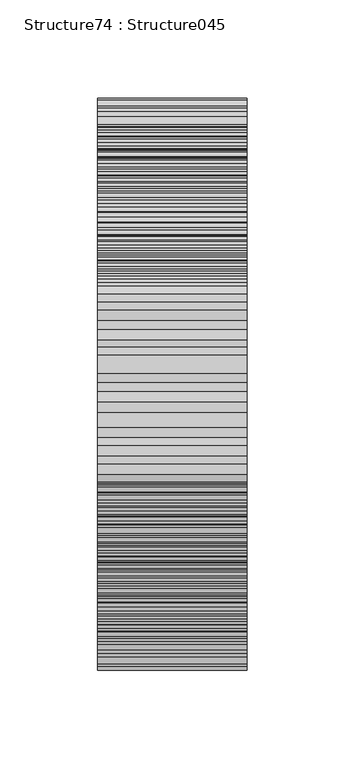
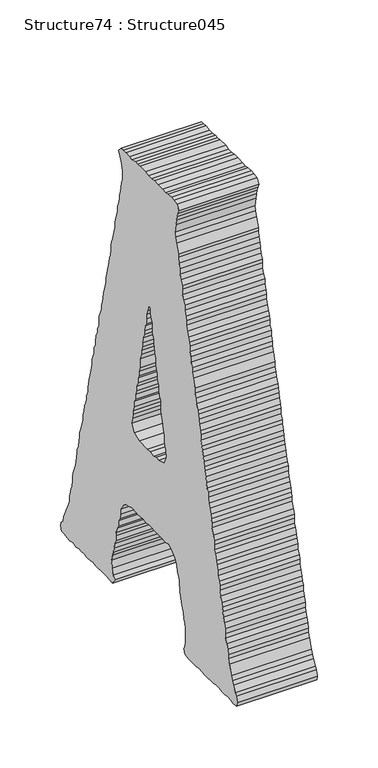
"""IFC4 building model written with IfcOpenShell, lengths in millimetres: proxy geometry, Structure74 : Structure045."""

from ifc_helpers import new_model, si_unit, frame, origin, place, context, project, spatial, polyline, outline, extrude, source, transform, mapped, element, save


def structure74_structure045_5a040be6(model_context):
    return source(origin(), model_context, "Body", "SweptSolid", [
        extrude(outline(polyline([(279560.8149563, 3818.8310229), (279560.8149563, 3814.7296538), (279561.9895268, 3811.2043377), (279564.3322494, 3805.9476534), (279564.3322494, 3801.8462843), (279564.9147208, 3795.960595), (279567.2558388, 3791.8865042), (279567.2558388, 3787.7867397), (279569.608189, 3783.0868532), (279570.1826374, 3777.8285642), (279570.1826374, 3773.11905), (279572.5317784, 3769.6274306), (279572.5317784, 3763.759392), (279574.2807973, 3759.6596275), (279576.0474668, 3755.559863), (279576.0474668, 3750.8583719), (279577.2156189, 3746.1745313), (279579.5679691, 3737.400554), (279580.7329119, 3732.1149867), (279581.8978548, 3727.4311462), (279583.0756345, 3723.3313817), (279583.0756345, 3718.6571688), (279584.8326764, 3713.3555556), (279585.4167525, 3709.2718371), (279587.1850266, 3704.5879966), (279588.3419465, 3701.0723082), (279588.9340455, 3695.786741), (279590.692692, 3690.512406), (279590.692692, 3685.8285655), (279591.8672625, 3682.8857208), (279593.0354146, 3677.6274319), (279594.8020842, 3672.9435914), (279596.5511031, 3668.8261762), (279597.1335745, 3664.1423357), (279597.7256735, 3660.0682449), (279598.3097496, 3654.1841602), (279600.6524721, 3650.1004418), (279601.233339, 3645.9830266), (279601.8270426, 3641.2991861), (279602.4175371, 3636.0408972), (279603.5760615, 3631.915459), (279605.3427311, 3627.8397636), (279607.1013776, 3622.555801), (279608.2679251, 3617.2718384), (279608.2679251, 3613.772196), (279608.8520011, 3607.8961343), (279610.6186707, 3604.3964919), (279611.7868227, 3600.2967274), (279612.9613932, 3595.5872132), (279613.5454693, 3589.7544759), (279614.7104121, 3586.2115092), (279618.8101766, 3577.4535778), (279621.1625268, 3572.1423369), (279622.9211733, 3568.6426945), (279624.0861162, 3563.366755), (279627.0209378, 3560.441561), (279628.1955083, 3556.3417965), (279626.4288388, 3551.6675836), (279621.7530213, 3551.6675836), (279617.0611577, 3551.0658569), (279612.9613932, 3550.4833855), (279607.6854537, 3551.6675836), (279602.4175371, 3550.4833855), (279597.7256735, 3551.6675836), (279594.2099851, 3551.0658569), (279588.3419465, 3551.6675836), (279584.8326764, 3551.0658569), (279578.9742654, 3551.0658569), (279574.8745009, 3551.6675836), (279570.7635042, 3551.0658569), (279566.0812683, 3551.0658569), (279561.3974278, 3551.6675836), (279552.0217237, 3551.6675836), (279547.3298602, 3551.0658569), (279542.0619436, 3550.4833855), (279538.5446505, 3556.3417965), (279541.4794722, 3559.2669905), (279543.2381187, 3565.1254015), (279543.8141717, 3572.7440636), (279542.0619436, 3578.6104977), (279540.295274, 3582.7102621), (279539.7128026, 3587.3860796), (279539.1383542, 3592.0955938), (279536.786004, 3596.7698067), (279536.786004, 3601.4536473), (279536.1955096, 3604.9709403), (279535.0289621, 3610.2292293), (279532.6798211, 3613.772196), (279532.1037681, 3619.6145609), (279530.3467262, 3622.555801), (279529.1689465, 3627.8397636), (279529.1689465, 3633.0980525), (279524.4867106, 3639.5405396), (279520.9613945, 3643.0578326), (279513.9348314, 3644.8245022), (279510.4175383, 3645.9830266), (279504.5591273, 3645.4262289), (279500.4577582, 3644.8245022), (279495.7674993, 3645.4262289), (279491.0820542, 3645.9830266), (279486.9919173, 3644.8245022), (279481.7063501, 3645.4262289), (279469.4070566, 3645.4262289), (279463.547041, 3644.8245022), (279454.1713369, 3644.8245022), (279449.4874964, 3645.9830266), (279443.0369864, 3642.4833842), (279438.9372219, 3638.9580681), (279436.0136325, 3633.0980525), (279434.8278298, 3627.2396415), (279433.0772062, 3622.555801), (279431.9042404, 3619.6145609), (279430.7360883, 3609.0723094), (279429.5695408, 3604.3964919), (279428.3949703, 3600.2967274), (279426.6347192, 3596.1953583), (279425.4601487, 3592.0955938), (279424.8760727, 3586.2115092), (279423.1190307, 3582.7102621), (279421.9444603, 3578.6104977), (279421.9444603, 3573.9266571), (279421.9444603, 3563.9412034), (279423.1190307, 3559.2669905), (279424.8760727, 3555.7416744), (279422.5365593, 3551.6675836), (279417.2590151, 3550.4833855), (279403.7851512, 3550.4833855), (279399.6837821, 3551.6675836), (279394.4094471, 3551.0658569), (279389.715979, 3550.4833855), (279385.6242375, 3550.4833855), (279379.7561989, 3551.0658569), (279375.6548298, 3551.0658569), (279370.9645708, 3551.6675836), (279366.8728294, 3551.6675836), (279362.1905934, 3550.4833855), (279356.9034216, 3550.4833855), (279352.2211857, 3551.6675836), (279346.9548738, 3551.0658569), (279343.4359761, 3550.4833855), (279337.5711467, 3551.0658569), (279336.4029946, 3555.1848766), (279338.1520135, 3560.441561), (279339.3378162, 3563.366755), (279342.8454816, 3568.6426945), (279344.6137558, 3572.1423369), (279346.3627747, 3576.2693797), (279349.2863641, 3586.2115092), (279351.0530336, 3590.3289243), (279351.0530336, 3594.4286888), (279352.2211857, 3599.1125293), (279353.3877332, 3604.3964919), (279355.7465018, 3608.4705827), (279356.3225548, 3612.5976255), (279356.3225548, 3617.2718384), (279357.4971253, 3622.555801), (279359.2557718, 3627.2396415), (279359.8382432, 3632.5155811), (279361.0047907, 3636.0408972), (279362.1905934, 3640.114988), (279363.9396123, 3645.4262289), (279365.1141828, 3650.6845178), (279365.1141828, 3655.3587307), (279366.2887533, 3659.4584952), (279368.6218483, 3663.5598643), (279368.6218483, 3668.8261762), (279370.3885178, 3673.5276674), (279370.9645708, 3677.0449604), (279372.7312404, 3682.8857208), (279373.9058109, 3686.4030139), (279373.9058109, 3691.0868544), (279374.4898869, 3695.2122926), (279375.6548298, 3699.8881101), (279378.00718, 3705.7545441), (279378.00718, 3710.4560353), (279379.1737274, 3714.5301261), (279380.3482979, 3718.0554422), (279381.5228684, 3723.3313817), (279383.2734919, 3727.4311462), (279384.449667, 3732.7167134), (279384.449667, 3737.9750024), (279386.1986859, 3740.9162424), (279387.3732564, 3745.6000829), (279387.9669601, 3751.4424479), (279389.715979, 3756.1423345), (279390.8905494, 3759.6596275), (279391.4746255, 3764.3611187), (279392.0667245, 3769.0176809), (279393.8157434, 3774.3032481), (279394.4094471, 3777.8285642), (279396.1680936, 3783.0868532), (279396.1680936, 3788.3611881), (279397.3330365, 3791.8865042), (279399.091683, 3797.1463977), (279399.6837821, 3801.8462843), (279400.8503296, 3806.5317294), (279401.4344056, 3810.0474179), (279403.7851512, 3815.3313805), (279404.950094, 3820.015221), (279406.1246645, 3824.1149855), (279406.1246645, 3829.374879), (279409.0514631, 3837.6000817), (279410.2260336, 3842.8583706), (279410.8181327, 3846.9757858), (279412.5687562, 3851.6612309), (279412.5687562, 3856.9179152), (279414.3257981, 3861.0192843), (279414.9195018, 3866.3032469), (279415.5003686, 3869.8189354), (279417.2590151, 3873.9203044), (279419.0192663, 3878.5784713), (279420.1858137, 3883.8881076), (279420.1858137, 3888.5623205), (279421.3603842, 3892.6636896), (279423.1190307, 3897.3475301), (279423.1190307, 3902.6314927), (279425.4601487, 3906.1487857), (279426.6347192, 3910.8310217), (279427.2107722, 3916.0909152), (279427.2107722, 3919.6066036), (279429.5695408, 3924.2888396), (279430.7360883, 3928.9919353), (279431.3201643, 3934.2758979), (279432.4947348, 3938.9517154), (279433.6709099, 3944.235678), (279433.6709099, 3947.1496398), (279437.188203, 3956.5349715), (279438.3435182, 3961.794865), (279439.5212979, 3965.8930249), (279437.7706744, 3974.7055128), (279436.5944993, 3979.9621971), (279436.0136325, 3983.4794902), (279434.8278298, 3987.5792547), (279432.4947348, 3991.6806238), (279436.0136325, 3996.390138), (279441.2879674, 3996.9645864), (279445.3893365, 3997.5486624), (279450.6556485, 3997.5486624), (279454.755413, 3996.390138), (279460.0393756, 3996.9645864), (279467.6564331, 3996.9645864), (279472.9147221, 3997.5486624), (279478.1986847, 3996.390138), (279482.8921528, 3996.390138), (279487.5647611, 3997.5486624), (279496.9404652, 3997.5486624), (279501.0514619, 3996.9645864), (279504.5591273, 3997.5486624), (279509.8366715, 3996.390138), (279514.5189074, 3996.390138), (279519.7932424, 3997.5486624), (279523.9026345, 3997.5486624), (279528.0040036, 3996.9645864), (279532.1037681, 3992.2614906), (279529.7530225, 3987.5792547), (279528.0040036, 3984.0635662), (279526.8294331, 3979.3781211), (279525.653258, 3974.7055128), (279525.653258, 3966.5043792), (279527.4102999, 3962.3757319), (279528.578452, 3957.1190475), (279529.1689465, 3952.435207), (279530.927593, 3947.7337158), (279530.927593, 3944.235678), (279532.1037681, 3938.3499888), (279533.8624146, 3934.8503464), (279533.8624146, 3929.5904528), (279535.6210611, 3924.8905662), (279537.37008, 3919.6066036), (279538.5446505, 3915.5068392), (279538.5446505, 3910.8310217), (279539.7128026, 3906.1487857), (279540.8873731, 3902.6314927), (279542.0619436, 3896.763454), (279543.8141717, 3893.822214), (279544.9887422, 3888.5623205), (279544.9887422, 3884.4609514), (279545.5808413, 3878.5784713), (279547.3298602, 3875.0772243), (279547.9123316, 3870.4030114), (279549.0981343, 3866.3032469), (279550.2630772, 3861.0192843), (279551.4312292, 3856.9179152), (279553.1978988, 3851.6612309), (279553.1978988, 3846.9757858), (279554.9469177, 3841.6741725), (279555.5293891, 3838.1761347), (279557.2960587, 3833.4730389), (279557.8801347, 3828.2163546), (279558.4642107, 3824.1149855), (279560.8149563, 3818.8310229)]), holes=[polyline([(279498.1262679, 3720.4158154), (279506.3177738, 3723.9154578), (279509.8366715, 3730.9323932), (279508.6685194, 3736.7988273), (279507.4939489, 3741.5003184), (279507.4939489, 3744.9999608), (279505.74493, 3750.3015741), (279505.74493, 3755.559863), (279503.9766559, 3759.0595054), (279503.3925799, 3764.3611187), (279502.2180094, 3768.4432325), (279502.2180094, 3773.11905), (279499.8768914, 3777.8285642), (279499.8768914, 3783.0868532), (279498.1262679, 3786.0280932), (279497.5341688, 3790.7039107), (279496.3595983, 3795.4037973), (279495.7674993, 3804.7730829), (279494.0168758, 3810.0474179), (279493.4327997, 3814.7296538), (279492.2582293, 3818.8310229), (279491.6661302, 3822.932392), (279491.0820542, 3828.790803), (279488.7425408, 3833.4730389), (279488.7425408, 3836.9919366), (279488.1488371, 3842.2758992), (279485.8157422, 3845.8012153), (279485.8157422, 3851.0595042), (279485.2252478, 3855.7353217), (279483.4649966, 3860.4432313), (279482.2984492, 3865.1190488), (279480.5317796, 3864.5446004), (279480.5317796, 3860.4432313), (279479.3748598, 3856.3161885), (279477.6081902, 3851.6612309), (279477.6081902, 3846.3772683), (279477.0241142, 3842.2758992), (279474.6813916, 3837.6000817), (279474.6813916, 3832.8921721), (279474.0892926, 3828.790803), (279472.9147221, 3824.1149855), (279471.7578022, 3819.4150989), (279471.1657032, 3813.5743386), (279470.5816271, 3810.0474179), (279468.813353, 3805.9476534), (279468.813353, 3800.6717138), (279466.472235, 3795.4037973), (279466.472235, 3790.7039107), (279465.2976645, 3786.0280932), (279463.547041, 3782.5027771), (279462.962965, 3777.2444882), (279462.962965, 3772.5606477), (279462.3724705, 3767.8607611), (279460.621847, 3763.759392), (279460.0393756, 3759.6596275), (279459.4472765, 3754.9854146), (279457.104554, 3750.8583719), (279457.6790024, 3744.9999608), (279456.5236871, 3740.9162424), (279455.3459074, 3736.7988273), (279454.1713369, 3730.9323932), (279457.104554, 3723.3313817), (279465.8897636, 3720.4158154), (279469.9911327, 3720.9726131), (279474.0892926, 3719.8140887), (279479.3748598, 3720.9726131), (279484.6411717, 3720.4158154), (279498.1262679, 3720.4158154)])]), frame((-59031.6926606, 0.0, 0.0), z_axis=(1.0, 0.0, 0.0), x_axis=(0.0, 1.0, 0.0)), (0.0, 0.0, 1.0), 76.2),
    ])


if __name__ == "__main__":
    model = new_model("IFC4")
    model_context = context("Model", 3, world=origin())
    ifc_project = project(units=[si_unit("LENGTHUNIT", "METRE", prefix="MILLI")], contexts=[model_context])
    site = spatial("IfcSite", under=ifc_project)
    building = spatial("IfcBuilding", under=site)
    placement = place(None, origin())
    structure74_structure045_shape = structure74_structure045_5a040be6(model_context)
    element("IfcBuildingElementProxy", 1, Name="Structure74 : Structure045", ObjectType="Structure74 : Structure045", at=placement, inside=building, context=model_context, shape_type="MappedRepresentation", body=[
        mapped(structure74_structure045_shape, transform((0.0, 0.0, 0.0), x_axis=(1.0, 0.0, 0.0), y_axis=(0.0, 1.0, 0.0), z_axis=(0.0, 0.0, 1.0))),
    ])
    save(model, "model.ifc")

# Revit data of these elements
# Type "Structure74 : Structure045"
#   NameOverride = "Structure045"
# Element 1 (IfcBuildingElementProxy, "Structure74 : Structure045")
#   Materials on its faces: "BRUSHED ALUM. LETTERING"
# Materials
#   "BRUSHED ALUM. LETTERING": class "Unassigned", colour RGB 169 181 186, transparency 0, Cost = 0
